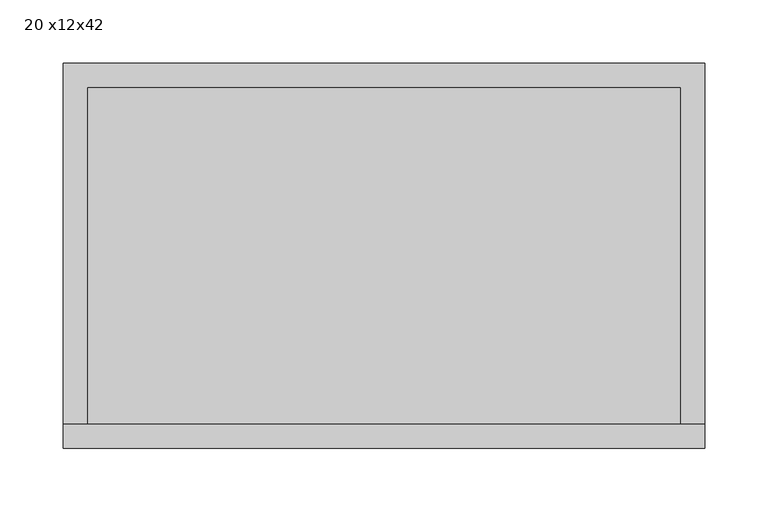
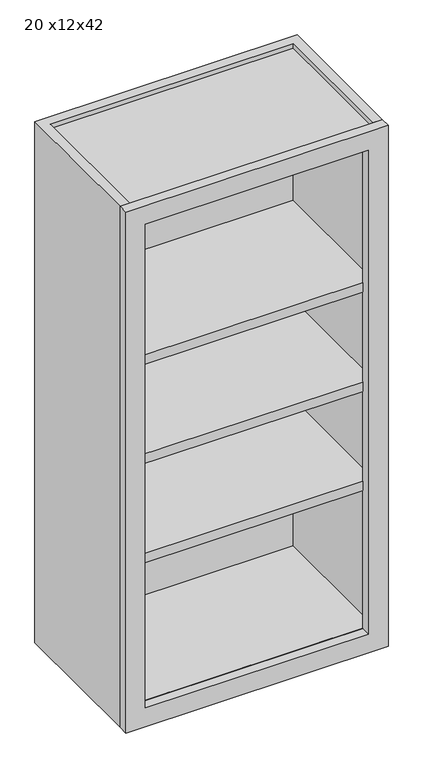
"""IFC4 building model written with IfcOpenShell, lengths in millimetres: furniture geometry, Bookcase-Merillat : 20 x12x42."""

import ifcopenshell
import ifcopenshell.guid

model = None  # the IFC model being written
_history = None  # IfcOwnerHistory: only IFC2X3 demands one
_inside = {}  # id of a spatial element -> (the spatial element, [elements in it])
_under = {}  # id of a project, library or spatial element -> (it, [spatial elements below it])
_declared = {}  # id of a project -> (the project, [libraries it declares])
_typed = {}  # id of a type object -> (the type object, [elements of that type])
_made_of = {}  # id of a material, layer set ... -> (it, [elements and type objects made of it])


def new_model(schema):
    """Start an empty IFC model of exactly this schema.

    Asked for "IFC4X3", IfcOpenShell would pick the latest addendum, in which some entities
    have other attributes; the version numbers below select the first issue.
    IFC2X3 requires an IfcOwnerHistory on every rooted entity: one is made here for all.
    """
    global model, _history
    if schema == "IFC4X3":
        model = ifcopenshell.file(schema_version=(4, 3, 0, 0))
    else:
        model = ifcopenshell.file(schema=schema)
    _inside.clear()
    _under.clear()
    _declared.clear()
    _typed.clear()
    _made_of.clear()
    _history = None
    if model.schema == "IFC2X3":
        org = make("IfcOrganization", Name="unknown")
        user = make(
            "IfcPersonAndOrganization",
            ThePerson=make("IfcPerson", FamilyName="unknown"),
            TheOrganization=org,
        )
        app = make(
            "IfcApplication",
            ApplicationDeveloper=org,
            Version="unknown",
            ApplicationFullName="unknown",
            ApplicationIdentifier="unknown",
        )
        _history = make(
            "IfcOwnerHistory",
            OwningUser=user,
            OwningApplication=app,
            ChangeAction="ADDED",
            CreationDate=0,
        )
    return model


def make(cls, **values):
    """One entity of the class cls with the attributes given. An attribute that is None is left unset."""
    return model.create_entity(
        cls, **{name: value for name, value in values.items() if value is not None}
    )


def rooted(cls, **values):
    """An entity with a GlobalId (a new one), such as an element, a storey or a relation."""
    return make(cls, GlobalId=ifcopenshell.guid.new(), OwnerHistory=_history, **values)


def si_unit(unit_type, name, prefix=None):
    """IfcSIUnit, for example si_unit("LENGTHUNIT", "METRE", prefix="MILLI")."""
    return make("IfcSIUnit", UnitType=unit_type, Prefix=prefix, Name=name)


def assignment(units):
    """IfcUnitAssignment: the units of a project."""
    return None if units is None else make("IfcUnitAssignment", Units=units)


def point(xyz):
    """IfcCartesianPoint."""
    return None if xyz is None else make("IfcCartesianPoint", Coordinates=xyz)


def direction(xyz):
    """IfcDirection."""
    return None if xyz is None else make("IfcDirection", DirectionRatios=xyz)


def frame(location, z_axis=None, x_axis=None):
    """IfcAxis2Placement3D, a coordinate frame: its origin and axes. An axis left out is left unset."""
    return make(
        "IfcAxis2Placement3D",
        Location=point(location),
        Axis=direction(z_axis),
        RefDirection=direction(x_axis),
    )


def origin():
    """The frame at (0, 0, 0) with its axes left unset."""
    return frame((0.0, 0.0, 0.0))


def place(relative_to, where):
    """IfcLocalPlacement: puts the frame where relative to a parent placement (None: the world)."""
    return make(
        "IfcLocalPlacement", PlacementRelTo=relative_to, RelativePlacement=where
    )


def context(
    kind, dimensions, precision=None, world=None, true_north=None, identifier=None
):
    """IfcGeometricRepresentationContext, for example the 3D "Model" context."""
    return make(
        "IfcGeometricRepresentationContext",
        ContextIdentifier=identifier,
        ContextType=kind,
        CoordinateSpaceDimension=dimensions,
        Precision=precision,
        WorldCoordinateSystem=world,
        TrueNorth=true_north,
    )


def project(units=None, contexts=None):
    """IfcProject with its units and contexts."""
    return rooted(
        "IfcProject",
        Name="project",
        RepresentationContexts=contexts,
        UnitsInContext=assignment(units),
    )


def spatial(cls, under=None, at=None, **own):
    """A site, building, storey or space (cls), placed at a placement, below another one or the project."""
    s = rooted(cls, ObjectPlacement=at, **own)
    if under is not None:
        _under.setdefault(under.id(), (under, []))[1].append(s)
    return s


def polyline(points):
    """IfcPolyline through the points."""
    return make("IfcPolyline", Points=[point(p) for p in points])


def outline(outer, holes=None, kind="AREA"):
    """IfcArbitraryClosedProfileDef: a profile drawn as a closed curve; with holes, ...WithVoids."""
    if holes is None:
        return make("IfcArbitraryClosedProfileDef", ProfileType=kind, OuterCurve=outer)
    return make(
        "IfcArbitraryProfileDefWithVoids",
        ProfileType=kind,
        OuterCurve=outer,
        InnerCurves=holes,
    )


def extrude(swept, where, along, depth):
    """IfcExtrudedAreaSolid: the profile swept, set in the frame where, extruded along a direction by depth."""
    return make(
        "IfcExtrudedAreaSolid",
        SweptArea=swept,
        Position=where,
        ExtrudedDirection=direction(along),
        Depth=depth,
    )


def faces_of(points, faces, orient=None, outer=None):
    """IfcFace entities. A face is a list of loops; a loop is a list of indices into points, from 0.

    orient and outer hold one flag for each loop. By default every Orientation is true, the
    first loop of a face is its IfcFaceOuterBound and the others are IfcFaceBound.
    """
    made = []
    for i, loops in enumerate(faces):
        bounds = []
        for j, loop in enumerate(loops):
            is_outer = j == 0 if outer is None else outer[i][j]
            bounds.append(
                make(
                    "IfcFaceOuterBound" if is_outer else "IfcFaceBound",
                    Bound=make("IfcPolyLoop", Polygon=[points[k] for k in loop]),
                    Orientation=True if orient is None else orient[i][j],
                )
            )
        made.append(make("IfcFace", Bounds=bounds))
    return made


def faceted_brep(points, faces, orient=None, outer=None, voids=None):
    """IfcFacetedBrep: a solid bounded by flat faces; with voids (closed shells), ...WithVoids."""
    shared = [point(p) for p in points]
    hull = make("IfcClosedShell", CfsFaces=faces_of(shared, faces, orient, outer))
    if voids is None:
        return make("IfcFacetedBrep", Outer=hull)
    return make(
        "IfcFacetedBrepWithVoids",
        Outer=hull,
        Voids=[
            make(cls, CfsFaces=faces_of(shared, fs, o, b)) for cls, fs, o, b in voids
        ],
    )


def shape(context_of_items, identifier, shape_type, items):
    """IfcShapeRepresentation: the items that make up one representation, for example the "Body"."""
    return make(
        "IfcShapeRepresentation",
        ContextOfItems=context_of_items,
        RepresentationIdentifier=identifier,
        RepresentationType=shape_type,
        Items=items,
    )


def source(mapping_origin, context_of_items, identifier, shape_type, items):
    """IfcRepresentationMap: a shape defined once, which mapped items show again and again."""
    return make(
        "IfcRepresentationMap",
        MappingOrigin=mapping_origin,
        MappedRepresentation=shape(context_of_items, identifier, shape_type, items),
    )


def transform(
    local_origin,
    x_axis=None,
    y_axis=None,
    z_axis=None,
    scale=None,
    scale2=None,
    scale3=None,
    uniform=True,
):
    """IfcCartesianTransformationOperator3D, or its non-uniform kind. x_axis, y_axis, z_axis: its Axis1, 2, 3."""
    if uniform:
        return make(
            "IfcCartesianTransformationOperator3D",
            Axis1=direction(x_axis),
            Axis2=direction(y_axis),
            LocalOrigin=point(local_origin),
            Scale=scale,
            Axis3=direction(z_axis),
        )
    return make(
        "IfcCartesianTransformationOperator3DnonUniform",
        Axis1=direction(x_axis),
        Axis2=direction(y_axis),
        LocalOrigin=point(local_origin),
        Scale=scale,
        Axis3=direction(z_axis),
        Scale2=scale2,
        Scale3=scale3,
    )


def mapped(mapping_source, mapping_target):
    """IfcMappedItem: shows the shape of a source again, moved by a transform."""
    return make(
        "IfcMappedItem", MappingSource=mapping_source, MappingTarget=mapping_target
    )


def made_of(thing, what):
    """Note that an element or type object is made of a material, layer set ...; save() writes the relation."""
    if what is not None:
        _made_of.setdefault(what.id(), (what, []))[1].append(thing)
    return thing


def element(
    cls,
    number,
    at=None,
    inside=None,
    cuts=None,
    type_object=None,
    material=None,
    context=None,
    identifier="Body",
    shape_type=None,
    held_by="IfcProductDefinitionShape",
    body=None,
    shapes=None,
    **own,
):
    """One element of the class cls, such as IfcWall. Its Tag is "e" and its number.

    at: its placement. inside: the storey or other place that contains it. cuts: it is an
    opening in that element (IfcRelVoidsElement). A single representation is given by context,
    identifier, shape_type and body (its items); several are given by shapes. held_by: the class
    of the entity that holds the representations. save() writes the other relations.
    """
    e = rooted(cls, Tag="e%d" % number, ObjectPlacement=at, **own)
    if body is not None:
        shapes = [shape(context, identifier, shape_type, body)]
    if shapes is not None:
        e.Representation = make(held_by, Representations=shapes)
    if inside is not None:
        _inside.setdefault(inside.id(), (inside, []))[1].append(e)
    if cuts is not None:
        rooted(
            "IfcRelVoidsElement", RelatingBuildingElement=cuts, RelatedOpeningElement=e
        )
    if type_object is not None:
        _typed.setdefault(type_object.id(), (type_object, []))[1].append(e)
    return made_of(e, material)


def aggregate(whole, parts):
    """IfcRelAggregates: a whole, such as a stair, and the parts it consists of."""
    return rooted("IfcRelAggregates", RelatingObject=whole, RelatedObjects=parts)


def save(model, path):
    """Write the relations noted so far, then the file.

    IfcRelAggregates (storeys below a building ...), IfcRelContainedInSpatialStructure (elements
    in a storey), IfcRelDefinesByType, IfcRelAssociatesMaterial and IfcRelDeclares: one each for
    every whole, place, type object, material and project.
    """
    for whole, parts in _under.values():
        aggregate(whole, parts)
    for where, things in _inside.values():
        rooted(
            "IfcRelContainedInSpatialStructure",
            RelatedElements=things,
            RelatingStructure=where,
        )
    for kind, things in _typed.values():
        rooted("IfcRelDefinesByType", RelatedObjects=things, RelatingType=kind)
    for what, things in _made_of.values():
        rooted("IfcRelAssociatesMaterial", RelatedObjects=things, RelatingMaterial=what)
    for by, libraries in _declared.values():
        rooted("IfcRelDeclares", RelatingContext=by, RelatedDefinitions=libraries)
    model.write(path)


def furniture_20_x12x42_f67bfd04(model_context):
    return source(origin(), model_context, "Body", "SolidModel", [
        extrude(outline(polyline([(-234.95, 133.35), (234.95, 133.35), (234.95, -133.35), (-234.95, -133.35), (-234.95, 133.35)])), frame((0.0, 0.0, 320.675), z_axis=(0.0, 0.0, 1.0), x_axis=(1.0, 0.0, 0.0)), (0.0, 0.0, 1.0), 19.3909952),
        extrude(outline(polyline([(-234.95, 133.35), (234.95, 133.35), (234.95, -133.35), (-234.95, -133.35), (-234.95, 133.35)])), frame((0.0, 0.0, 726.7340048), z_axis=(0.0, 0.0, 1.0), x_axis=(1.0, 0.0, 0.0)), (0.0, 0.0, 1.0), 19.3909952),
        extrude(outline(polyline([(-234.95, 133.35), (234.95, 133.35), (234.95, -133.35), (-234.95, -133.35), (-234.95, 133.35)])), frame((0.0, 0.0, 523.7180074), z_axis=(0.0, 0.0, 1.0), x_axis=(1.0, 0.0, 0.0)), (0.0, 0.0, 1.0), 19.3909952),
        extrude(outline(polyline([(-234.95, 133.35), (234.95, 133.35), (234.95, -133.35), (-234.95, -133.35), (-234.95, 133.35)])), frame((0.0, 0.0, 19.3909952), z_axis=(0.0, 0.0, 1.0), x_axis=(1.0, 0.0, 0.0)), (0.0, 0.0, 1.0), 19.3909952),
        extrude(outline(polyline([(0.0, -254.0), (0.0, 254.0), (1066.8, 254.0), (1066.8, -254.0), (0.0, -254.0)]), holes=[polyline([(1028.7, -215.9), (1028.7, 215.9), (38.1, 215.9), (38.1, -215.9), (1028.7, -215.9)])]), frame((0.0, -152.4, 0.0), z_axis=(0.0, 1.0, 0.0), x_axis=(0.0, 0.0, 1.0)), (0.0, 0.0, 1.0), 19.05),
        faceted_brep([(-234.95, -133.35, 19.3909952), (234.95, -133.35, 19.3909952), (234.95, 133.35, 19.3909952), (-234.95, 133.35, 19.3909952), (-254.0, 152.4, 0.0), (254.0, 152.4, 0.0), (254.0, -133.35, 0.0), (-254.0, -133.35, 0.0), (-254.0, -133.35, 1066.8), (254.0, -133.35, 1066.8), (234.95, -133.35, 1066.8), (234.95, -133.35, 1057.5909423), (-234.95, -133.35, 1057.5909423), (-234.95, -133.35, 1066.8), (-234.95, -133.35, 1047.4090048), (234.95, -133.35, 1047.4090048), (-234.95, 133.35, 1057.5909423), (234.95, 133.35, 1057.5909423), (-234.95, 133.35, 1066.8), (234.95, 133.35, 1066.8), (-254.0, 152.4, 1066.8), (254.0, 152.4, 1066.8), (-234.95, 133.35, 1047.4090048), (234.95, 133.35, 1047.4090048)], [[[0, 1, 2, 3]], [[4, 5, 6, 7]], [[8, 7, 6, 9, 10, 11, 12, 13], [1, 0, 14, 15]], [[16, 12, 11, 17]], [[12, 16, 18, 13]], [[17, 11, 10, 19]], [[16, 17, 19, 18]], [[20, 8, 13, 18, 19, 10, 9, 21]], [[8, 20, 4, 7]], [[0, 3, 22, 14]], [[3, 2, 23, 22]], [[2, 1, 15, 23]], [[21, 9, 6, 5]], [[20, 21, 5, 4]], [[15, 14, 22, 23]]]),
    ])


if __name__ == "__main__":
    model = new_model("IFC4")
    model_context = context("Model", 3, world=origin())
    ifc_project = project(units=[si_unit("LENGTHUNIT", "METRE", prefix="MILLI")], contexts=[model_context])
    site = spatial("IfcSite", under=ifc_project)
    building = spatial("IfcBuilding", under=site)
    placement = place(None, origin())
    furniture_20_x12x42_shape = furniture_20_x12x42_f67bfd04(model_context)
    element("IfcFurniture", 1, ObjectType="Bookcase-Merillat : 20 x12x42", at=placement, inside=building, context=model_context, shape_type="MappedRepresentation", body=[
        mapped(furniture_20_x12x42_shape, transform((0.0, 0.0, 0.0), x_axis=(1.0, 0.0, 0.0), y_axis=(0.0, 1.0, 0.0), z_axis=(0.0, 0.0, 1.0))),
    ])
    save(model, "model.ifc")

# Revit data of these elements
# Type "Bookcase-Merillat : 20 x12x42"
#   URL = "https://www.merillat.com/"
#   Product Page URL = "https://www.merillat.com/our-products/"
#   Product Documentation Link = "http://merillatbusiness.com/wp-content/uploads/2014/07/Merillat_Classic_Catalog.pdf"
#   Model = "BK2136"
#   Manufacturer = "Merillat"
#   Description = "Bookcase"
#   Construction Type = "Bookcase"
#   Assembly Code = "E2020200"
#   Width = 1' - 8"
#   Shelving Height = 1' - 1"
#   Height = 3' - 6"
#   Depth = 1' - 0"
#   Default Elevation = 4' - 0"
#   Cabinet Shell = 0' - 0 3/4"
#   COBie.Type = no
#   Two Drawer = yes
#   Shelves Bookcase = yes
#   Number of Shelves = 2
#   No Shelf Bookcase = no
#   Middle Shelf = yes
#   Shelving Material = Wood - Merillat - Pecan(1)
#   Bookcase Material = Wood - Merillat - Pecan(1)
# Element 1 (IfcFurniture, "Bookcase-Merillat : 20 x12x42")
#   Materials on its faces: "Wood - Merillat - Pecan(1)"
# Materials
#   "Wood - Merillat - Pecan(1)": class "Wood", colour RGB 108 67 43, transparency 0, Cost = 0
